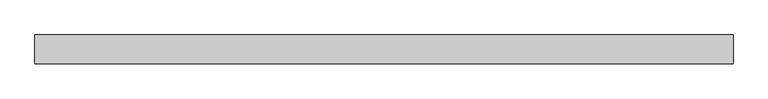
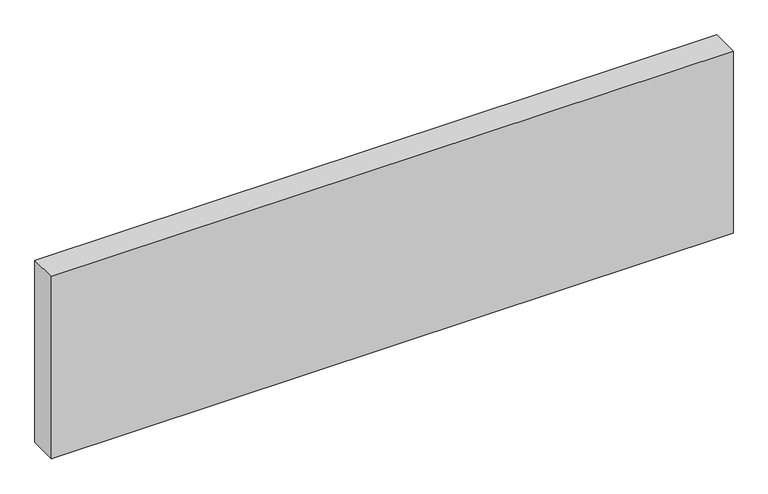
"""IFC4 building model written with IfcOpenShell, lengths in millimetres: proxy geometry, Generic Models 7:Generic Models 1:6:Generic Models 1:6 : Generic Models 7:Generic Models 1:337419:5 : Generic Models 7:Generic Models 1:6:Generic Models 1:6 : Generic Models 7:Generic Models 1:337419:312901."""

from ifc_helpers import new_model, si_unit, frame, origin, place, context, project, spatial, polyline, outline, extrude, source, transform, mapped, element, save


def generic_models_851fe7a5(model_context):
    return source(origin(), model_context, "Body", "SweptSolid", [
        extrude(outline(polyline([(596182.8367242, -536557.2913358), (596182.8367242, -536760.4913358), (591306.0367242, -536760.4913358), (591306.0367242, -536557.2913358), (596182.8367242, -536557.2913358)])), frame((0.0, 0.0, -1377.3372439), z_axis=(0.0, 0.0, 1.0), x_axis=(1.0, 0.0, 0.0)), (0.0, 0.0, 1.0), 1377.3372439),
    ])


if __name__ == "__main__":
    model = new_model("IFC4")
    model_context = context("Model", 3, world=origin())
    ifc_project = project(units=[si_unit("LENGTHUNIT", "METRE", prefix="MILLI")], contexts=[model_context])
    site = spatial("IfcSite", under=ifc_project)
    building = spatial("IfcBuilding", under=site)
    placement = place(None, origin())
    generic_models_shape = generic_models_851fe7a5(model_context)
    element("IfcBuildingElementProxy", 1, Name="Generic Models 7:Generic Models 1:6:Generic Models 1:6 : Generic Models 7:Generic Models 1:337419:5 : Generic Models 7:Generic Models 1:6:Generic Models 1:6 : Generic Models 7:Generic Models 1:337419:312901", ObjectType="Generic Models 7:Generic Models 1:6:Generic Models 1:6 : Generic Models 7:Generic Models 1:337419:5 : Generic Models 7:Generic Models 1:6:Generic Models 1:6 : Generic Models 7:Generic Models 1:337419:312901", at=placement, inside=building, context=model_context, shape_type="MappedRepresentation", body=[
        mapped(generic_models_shape, transform((0.0, 0.0, 0.0), x_axis=(1.0, 0.0, 0.0), y_axis=(0.0, 1.0, 0.0), z_axis=(0.0, 0.0, 1.0))),
    ])
    save(model, "model.ifc")

# Revit data of these elements
# Type "Generic Models 7:Generic Models 1:6:Generic Models 1:6 : Generic Models 7:Generic Models 1:337419:5 : Generic Models 7:Generic Models 1:6:Generic Models 1:6 : Generic Models 7:Generic Models 1:337419:312901"
#   NameOverride = "Generic Models 7:Generic Models 1:6:Generic Models 1:6 : Generic Models 7:Generic Models 1:337419:312901"
#   ObjectTypeOverride = "Generic Models 1:6 : Generic Models 7:Generic Models 1:337419"
#   Reference = "Generic Models 1"
#   Tag = "312901"
# Element 1 (IfcBuildingElementProxy, "Generic Models 7:Generic Models 1:6:Generic Models 1:6 : Generic Models 7:Generic Models 1:337419:5 : Generic Models 7:Generic Models 1:6:Generic Models 1:6 : Generic Models 7:Generic Models 1:337419:312901")
#   Materials on its faces: "CONCRETE FROST WALL - SEE STRUCT DWGS."
# Materials
#   "CONCRETE FROST WALL - SEE STRUCT DWGS.": class "Concrete", colour RGB 115 116 108, transparency 0, Description = "Lightweight concrete", Cost = 0
